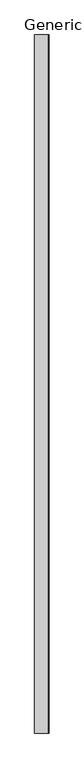
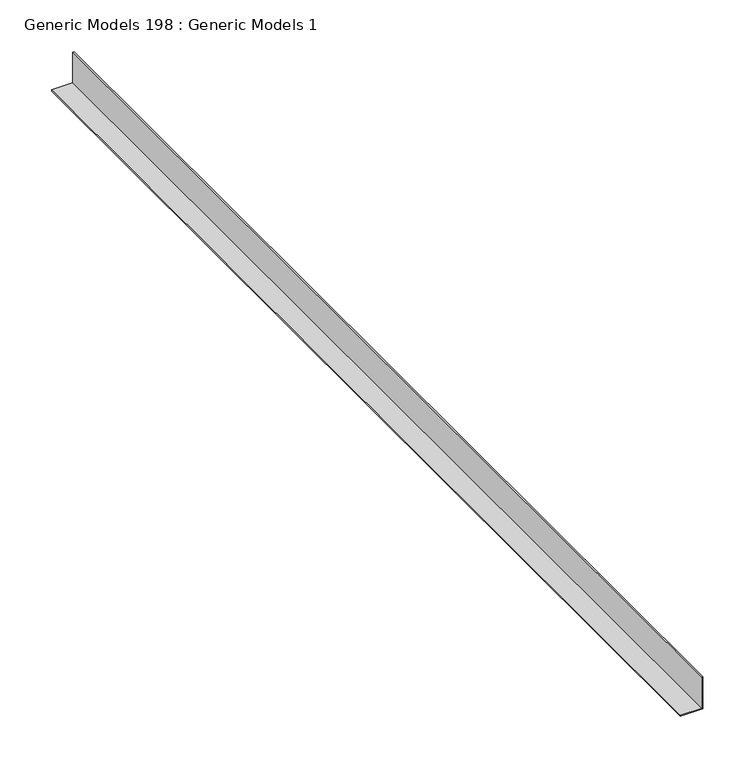
"""IFC4 building model written with IfcOpenShell, lengths in millimetres: proxy geometry, Generic Models 198 : Generic Models 1."""

import ifcopenshell
import ifcopenshell.guid

model = None  # the IFC model being written
_history = None  # IfcOwnerHistory: only IFC2X3 demands one
_inside = {}  # id of a spatial element -> (the spatial element, [elements in it])
_under = {}  # id of a project, library or spatial element -> (it, [spatial elements below it])
_declared = {}  # id of a project -> (the project, [libraries it declares])
_typed = {}  # id of a type object -> (the type object, [elements of that type])
_made_of = {}  # id of a material, layer set ... -> (it, [elements and type objects made of it])


def new_model(schema):
    """Start an empty IFC model of exactly this schema.

    Asked for "IFC4X3", IfcOpenShell would pick the latest addendum, in which some entities
    have other attributes; the version numbers below select the first issue.
    IFC2X3 requires an IfcOwnerHistory on every rooted entity: one is made here for all.
    """
    global model, _history
    if schema == "IFC4X3":
        model = ifcopenshell.file(schema_version=(4, 3, 0, 0))
    else:
        model = ifcopenshell.file(schema=schema)
    _inside.clear()
    _under.clear()
    _declared.clear()
    _typed.clear()
    _made_of.clear()
    _history = None
    if model.schema == "IFC2X3":
        org = make("IfcOrganization", Name="unknown")
        user = make(
            "IfcPersonAndOrganization",
            ThePerson=make("IfcPerson", FamilyName="unknown"),
            TheOrganization=org,
        )
        app = make(
            "IfcApplication",
            ApplicationDeveloper=org,
            Version="unknown",
            ApplicationFullName="unknown",
            ApplicationIdentifier="unknown",
        )
        _history = make(
            "IfcOwnerHistory",
            OwningUser=user,
            OwningApplication=app,
            ChangeAction="ADDED",
            CreationDate=0,
        )
    return model


def make(cls, **values):
    """One entity of the class cls with the attributes given. An attribute that is None is left unset."""
    return model.create_entity(
        cls, **{name: value for name, value in values.items() if value is not None}
    )


def rooted(cls, **values):
    """An entity with a GlobalId (a new one), such as an element, a storey or a relation."""
    return make(cls, GlobalId=ifcopenshell.guid.new(), OwnerHistory=_history, **values)


def si_unit(unit_type, name, prefix=None):
    """IfcSIUnit, for example si_unit("LENGTHUNIT", "METRE", prefix="MILLI")."""
    return make("IfcSIUnit", UnitType=unit_type, Prefix=prefix, Name=name)


def assignment(units):
    """IfcUnitAssignment: the units of a project."""
    return None if units is None else make("IfcUnitAssignment", Units=units)


def point(xyz):
    """IfcCartesianPoint."""
    return None if xyz is None else make("IfcCartesianPoint", Coordinates=xyz)


def direction(xyz):
    """IfcDirection."""
    return None if xyz is None else make("IfcDirection", DirectionRatios=xyz)


def frame(location, z_axis=None, x_axis=None):
    """IfcAxis2Placement3D, a coordinate frame: its origin and axes. An axis left out is left unset."""
    return make(
        "IfcAxis2Placement3D",
        Location=point(location),
        Axis=direction(z_axis),
        RefDirection=direction(x_axis),
    )


def origin():
    """The frame at (0, 0, 0) with its axes left unset."""
    return frame((0.0, 0.0, 0.0))


def place(relative_to, where):
    """IfcLocalPlacement: puts the frame where relative to a parent placement (None: the world)."""
    return make(
        "IfcLocalPlacement", PlacementRelTo=relative_to, RelativePlacement=where
    )


def context(
    kind, dimensions, precision=None, world=None, true_north=None, identifier=None
):
    """IfcGeometricRepresentationContext, for example the 3D "Model" context."""
    return make(
        "IfcGeometricRepresentationContext",
        ContextIdentifier=identifier,
        ContextType=kind,
        CoordinateSpaceDimension=dimensions,
        Precision=precision,
        WorldCoordinateSystem=world,
        TrueNorth=true_north,
    )


def project(units=None, contexts=None):
    """IfcProject with its units and contexts."""
    return rooted(
        "IfcProject",
        Name="project",
        RepresentationContexts=contexts,
        UnitsInContext=assignment(units),
    )


def spatial(cls, under=None, at=None, **own):
    """A site, building, storey or space (cls), placed at a placement, below another one or the project."""
    s = rooted(cls, ObjectPlacement=at, **own)
    if under is not None:
        _under.setdefault(under.id(), (under, []))[1].append(s)
    return s


def polyline(points):
    """IfcPolyline through the points."""
    return make("IfcPolyline", Points=[point(p) for p in points])


def outline(outer, holes=None, kind="AREA"):
    """IfcArbitraryClosedProfileDef: a profile drawn as a closed curve; with holes, ...WithVoids."""
    if holes is None:
        return make("IfcArbitraryClosedProfileDef", ProfileType=kind, OuterCurve=outer)
    return make(
        "IfcArbitraryProfileDefWithVoids",
        ProfileType=kind,
        OuterCurve=outer,
        InnerCurves=holes,
    )


def extrude(swept, where, along, depth):
    """IfcExtrudedAreaSolid: the profile swept, set in the frame where, extruded along a direction by depth."""
    return make(
        "IfcExtrudedAreaSolid",
        SweptArea=swept,
        Position=where,
        ExtrudedDirection=direction(along),
        Depth=depth,
    )


def shape(context_of_items, identifier, shape_type, items):
    """IfcShapeRepresentation: the items that make up one representation, for example the "Body"."""
    return make(
        "IfcShapeRepresentation",
        ContextOfItems=context_of_items,
        RepresentationIdentifier=identifier,
        RepresentationType=shape_type,
        Items=items,
    )


def source(mapping_origin, context_of_items, identifier, shape_type, items):
    """IfcRepresentationMap: a shape defined once, which mapped items show again and again."""
    return make(
        "IfcRepresentationMap",
        MappingOrigin=mapping_origin,
        MappedRepresentation=shape(context_of_items, identifier, shape_type, items),
    )


def transform(
    local_origin,
    x_axis=None,
    y_axis=None,
    z_axis=None,
    scale=None,
    scale2=None,
    scale3=None,
    uniform=True,
):
    """IfcCartesianTransformationOperator3D, or its non-uniform kind. x_axis, y_axis, z_axis: its Axis1, 2, 3."""
    if uniform:
        return make(
            "IfcCartesianTransformationOperator3D",
            Axis1=direction(x_axis),
            Axis2=direction(y_axis),
            LocalOrigin=point(local_origin),
            Scale=scale,
            Axis3=direction(z_axis),
        )
    return make(
        "IfcCartesianTransformationOperator3DnonUniform",
        Axis1=direction(x_axis),
        Axis2=direction(y_axis),
        LocalOrigin=point(local_origin),
        Scale=scale,
        Axis3=direction(z_axis),
        Scale2=scale2,
        Scale3=scale3,
    )


def mapped(mapping_source, mapping_target):
    """IfcMappedItem: shows the shape of a source again, moved by a transform."""
    return make(
        "IfcMappedItem", MappingSource=mapping_source, MappingTarget=mapping_target
    )


def made_of(thing, what):
    """Note that an element or type object is made of a material, layer set ...; save() writes the relation."""
    if what is not None:
        _made_of.setdefault(what.id(), (what, []))[1].append(thing)
    return thing


def element(
    cls,
    number,
    at=None,
    inside=None,
    cuts=None,
    type_object=None,
    material=None,
    context=None,
    identifier="Body",
    shape_type=None,
    held_by="IfcProductDefinitionShape",
    body=None,
    shapes=None,
    **own,
):
    """One element of the class cls, such as IfcWall. Its Tag is "e" and its number.

    at: its placement. inside: the storey or other place that contains it. cuts: it is an
    opening in that element (IfcRelVoidsElement). A single representation is given by context,
    identifier, shape_type and body (its items); several are given by shapes. held_by: the class
    of the entity that holds the representations. save() writes the other relations.
    """
    e = rooted(cls, Tag="e%d" % number, ObjectPlacement=at, **own)
    if body is not None:
        shapes = [shape(context, identifier, shape_type, body)]
    if shapes is not None:
        e.Representation = make(held_by, Representations=shapes)
    if inside is not None:
        _inside.setdefault(inside.id(), (inside, []))[1].append(e)
    if cuts is not None:
        rooted(
            "IfcRelVoidsElement", RelatingBuildingElement=cuts, RelatedOpeningElement=e
        )
    if type_object is not None:
        _typed.setdefault(type_object.id(), (type_object, []))[1].append(e)
    return made_of(e, material)


def aggregate(whole, parts):
    """IfcRelAggregates: a whole, such as a stair, and the parts it consists of."""
    return rooted("IfcRelAggregates", RelatingObject=whole, RelatedObjects=parts)


def save(model, path):
    """Write the relations noted so far, then the file.

    IfcRelAggregates (storeys below a building ...), IfcRelContainedInSpatialStructure (elements
    in a storey), IfcRelDefinesByType, IfcRelAssociatesMaterial and IfcRelDeclares: one each for
    every whole, place, type object, material and project.
    """
    for whole, parts in _under.values():
        aggregate(whole, parts)
    for where, things in _inside.values():
        rooted(
            "IfcRelContainedInSpatialStructure",
            RelatedElements=things,
            RelatingStructure=where,
        )
    for kind, things in _typed.values():
        rooted("IfcRelDefinesByType", RelatedObjects=things, RelatingType=kind)
    for what, things in _made_of.values():
        rooted("IfcRelAssociatesMaterial", RelatedObjects=things, RelatingMaterial=what)
    for by, libraries in _declared.values():
        rooted("IfcRelDeclares", RelatingContext=by, RelatedDefinitions=libraries)
    model.write(path)


def generic_models_198_generic_models_1_f99cc74d(model_context):
    return source(origin(), model_context, "Body", "SweptSolid", [
        extrude(outline(polyline([(2277.1204978, 49676.05), (2277.1204978, 49674.4625), (2240.6079978, 49674.4625), (2240.6079978, 49650.65), (2239.0204978, 49650.65), (2239.0204978, 49676.05), (2277.1204978, 49676.05)])), frame((0.0, 0.0, 0.0), z_axis=(0.0, 1.0, 0.0), x_axis=(0.0, 0.0, 1.0)), (0.0, 0.0, 1.0), 1219.2),
    ])


if __name__ == "__main__":
    model = new_model("IFC4")
    model_context = context("Model", 3, world=origin())
    ifc_project = project(units=[si_unit("LENGTHUNIT", "METRE", prefix="MILLI")], contexts=[model_context])
    site = spatial("IfcSite", under=ifc_project)
    building = spatial("IfcBuilding", under=site)
    placement = place(None, origin())
    generic_models_198_generic_models_1_shape = generic_models_198_generic_models_1_f99cc74d(model_context)
    element("IfcBuildingElementProxy", 1, Name="Generic Models 198 : Generic Models 1", ObjectType="Generic Models 198 : Generic Models 1", at=placement, inside=building, context=model_context, shape_type="MappedRepresentation", body=[
        mapped(generic_models_198_generic_models_1_shape, transform((0.0, 0.0, 0.0), x_axis=(1.0, 0.0, 0.0), y_axis=(0.0, 1.0, 0.0), z_axis=(0.0, 0.0, 1.0))),
    ])
    save(model, "model.ifc")

# Revit data of these elements
# Element 1 (IfcBuildingElementProxy, "Generic Models 198 : Generic Models 1")
#   Materials on its faces: "CEILING TRACK AS SCHEDULED"
# Materials
#   "CEILING TRACK AS SCHEDULED": class "Unassigned", colour RGB 210 209 208, transparency 0, Keynote = "M05121300.02", Cost = 0
